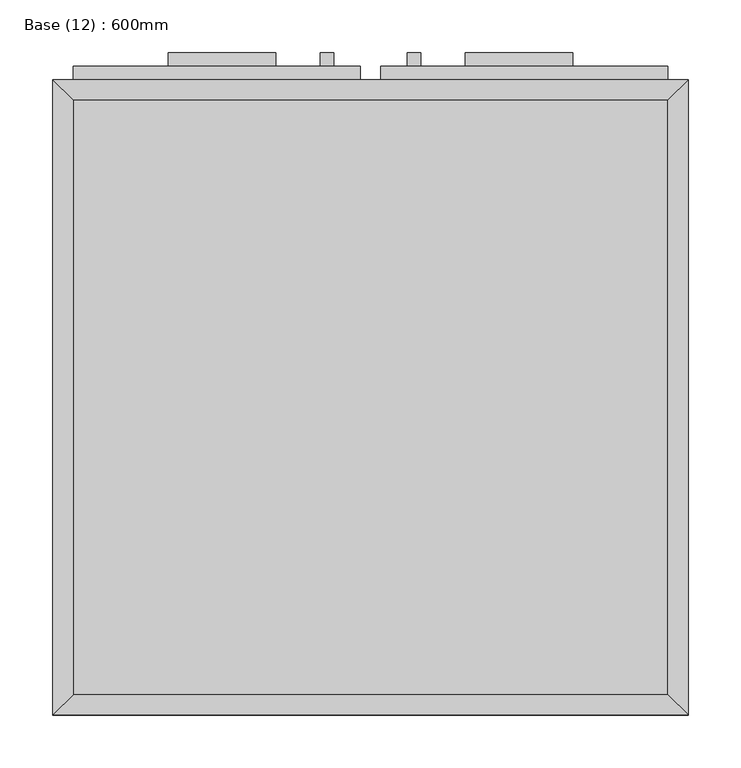
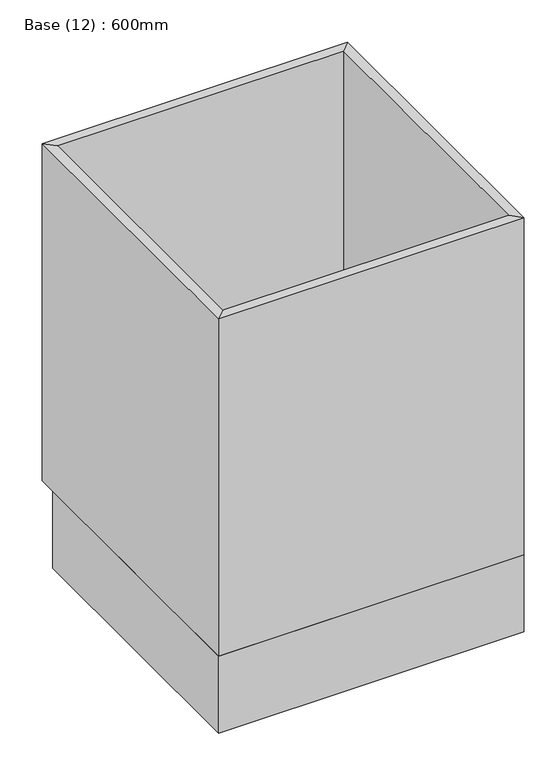
"""IFC4 building model written with IfcOpenShell, lengths in millimetres: furniture geometry, Base (12) : 600mm."""

import ifcopenshell
import ifcopenshell.guid

model = None  # the IFC model being written
_history = None  # IfcOwnerHistory: only IFC2X3 demands one
_inside = {}  # id of a spatial element -> (the spatial element, [elements in it])
_under = {}  # id of a project, library or spatial element -> (it, [spatial elements below it])
_declared = {}  # id of a project -> (the project, [libraries it declares])
_typed = {}  # id of a type object -> (the type object, [elements of that type])
_made_of = {}  # id of a material, layer set ... -> (it, [elements and type objects made of it])


def new_model(schema):
    """Start an empty IFC model of exactly this schema.

    Asked for "IFC4X3", IfcOpenShell would pick the latest addendum, in which some entities
    have other attributes; the version numbers below select the first issue.
    IFC2X3 requires an IfcOwnerHistory on every rooted entity: one is made here for all.
    """
    global model, _history
    if schema == "IFC4X3":
        model = ifcopenshell.file(schema_version=(4, 3, 0, 0))
    else:
        model = ifcopenshell.file(schema=schema)
    _inside.clear()
    _under.clear()
    _declared.clear()
    _typed.clear()
    _made_of.clear()
    _history = None
    if model.schema == "IFC2X3":
        org = make("IfcOrganization", Name="unknown")
        user = make(
            "IfcPersonAndOrganization",
            ThePerson=make("IfcPerson", FamilyName="unknown"),
            TheOrganization=org,
        )
        app = make(
            "IfcApplication",
            ApplicationDeveloper=org,
            Version="unknown",
            ApplicationFullName="unknown",
            ApplicationIdentifier="unknown",
        )
        _history = make(
            "IfcOwnerHistory",
            OwningUser=user,
            OwningApplication=app,
            ChangeAction="ADDED",
            CreationDate=0,
        )
    return model


def make(cls, **values):
    """One entity of the class cls with the attributes given. An attribute that is None is left unset."""
    return model.create_entity(
        cls, **{name: value for name, value in values.items() if value is not None}
    )


def rooted(cls, **values):
    """An entity with a GlobalId (a new one), such as an element, a storey or a relation."""
    return make(cls, GlobalId=ifcopenshell.guid.new(), OwnerHistory=_history, **values)


def si_unit(unit_type, name, prefix=None):
    """IfcSIUnit, for example si_unit("LENGTHUNIT", "METRE", prefix="MILLI")."""
    return make("IfcSIUnit", UnitType=unit_type, Prefix=prefix, Name=name)


def assignment(units):
    """IfcUnitAssignment: the units of a project."""
    return None if units is None else make("IfcUnitAssignment", Units=units)


def point(xyz):
    """IfcCartesianPoint."""
    return None if xyz is None else make("IfcCartesianPoint", Coordinates=xyz)


def direction(xyz):
    """IfcDirection."""
    return None if xyz is None else make("IfcDirection", DirectionRatios=xyz)


def frame(location, z_axis=None, x_axis=None):
    """IfcAxis2Placement3D, a coordinate frame: its origin and axes. An axis left out is left unset."""
    return make(
        "IfcAxis2Placement3D",
        Location=point(location),
        Axis=direction(z_axis),
        RefDirection=direction(x_axis),
    )


def origin():
    """The frame at (0, 0, 0) with its axes left unset."""
    return frame((0.0, 0.0, 0.0))


def origin_with_axes():
    """The frame at (0, 0, 0) with the z axis (0, 0, 1) and the x axis (1, 0, 0) written out."""
    return frame((0.0, 0.0, 0.0), z_axis=(0.0, 0.0, 1.0), x_axis=(1.0, 0.0, 0.0))


def place(relative_to, where):
    """IfcLocalPlacement: puts the frame where relative to a parent placement (None: the world)."""
    return make(
        "IfcLocalPlacement", PlacementRelTo=relative_to, RelativePlacement=where
    )


def context(
    kind, dimensions, precision=None, world=None, true_north=None, identifier=None
):
    """IfcGeometricRepresentationContext, for example the 3D "Model" context."""
    return make(
        "IfcGeometricRepresentationContext",
        ContextIdentifier=identifier,
        ContextType=kind,
        CoordinateSpaceDimension=dimensions,
        Precision=precision,
        WorldCoordinateSystem=world,
        TrueNorth=true_north,
    )


def project(units=None, contexts=None):
    """IfcProject with its units and contexts."""
    return rooted(
        "IfcProject",
        Name="project",
        RepresentationContexts=contexts,
        UnitsInContext=assignment(units),
    )


def spatial(cls, under=None, at=None, **own):
    """A site, building, storey or space (cls), placed at a placement, below another one or the project."""
    s = rooted(cls, ObjectPlacement=at, **own)
    if under is not None:
        _under.setdefault(under.id(), (under, []))[1].append(s)
    return s


def polyline(points):
    """IfcPolyline through the points."""
    return make("IfcPolyline", Points=[point(p) for p in points])


def outline(outer, holes=None, kind="AREA"):
    """IfcArbitraryClosedProfileDef: a profile drawn as a closed curve; with holes, ...WithVoids."""
    if holes is None:
        return make("IfcArbitraryClosedProfileDef", ProfileType=kind, OuterCurve=outer)
    return make(
        "IfcArbitraryProfileDefWithVoids",
        ProfileType=kind,
        OuterCurve=outer,
        InnerCurves=holes,
    )


def extrude(swept, where, along, depth):
    """IfcExtrudedAreaSolid: the profile swept, set in the frame where, extruded along a direction by depth."""
    return make(
        "IfcExtrudedAreaSolid",
        SweptArea=swept,
        Position=where,
        ExtrudedDirection=direction(along),
        Depth=depth,
    )


def faces_of(points, faces, orient=None, outer=None):
    """IfcFace entities. A face is a list of loops; a loop is a list of indices into points, from 0.

    orient and outer hold one flag for each loop. By default every Orientation is true, the
    first loop of a face is its IfcFaceOuterBound and the others are IfcFaceBound.
    """
    made = []
    for i, loops in enumerate(faces):
        bounds = []
        for j, loop in enumerate(loops):
            is_outer = j == 0 if outer is None else outer[i][j]
            bounds.append(
                make(
                    "IfcFaceOuterBound" if is_outer else "IfcFaceBound",
                    Bound=make("IfcPolyLoop", Polygon=[points[k] for k in loop]),
                    Orientation=True if orient is None else orient[i][j],
                )
            )
        made.append(make("IfcFace", Bounds=bounds))
    return made


def faceted_brep(points, faces, orient=None, outer=None, voids=None):
    """IfcFacetedBrep: a solid bounded by flat faces; with voids (closed shells), ...WithVoids."""
    shared = [point(p) for p in points]
    hull = make("IfcClosedShell", CfsFaces=faces_of(shared, faces, orient, outer))
    if voids is None:
        return make("IfcFacetedBrep", Outer=hull)
    return make(
        "IfcFacetedBrepWithVoids",
        Outer=hull,
        Voids=[
            make(cls, CfsFaces=faces_of(shared, fs, o, b)) for cls, fs, o, b in voids
        ],
    )


def shape(context_of_items, identifier, shape_type, items):
    """IfcShapeRepresentation: the items that make up one representation, for example the "Body"."""
    return make(
        "IfcShapeRepresentation",
        ContextOfItems=context_of_items,
        RepresentationIdentifier=identifier,
        RepresentationType=shape_type,
        Items=items,
    )


def source(mapping_origin, context_of_items, identifier, shape_type, items):
    """IfcRepresentationMap: a shape defined once, which mapped items show again and again."""
    return make(
        "IfcRepresentationMap",
        MappingOrigin=mapping_origin,
        MappedRepresentation=shape(context_of_items, identifier, shape_type, items),
    )


def transform(
    local_origin,
    x_axis=None,
    y_axis=None,
    z_axis=None,
    scale=None,
    scale2=None,
    scale3=None,
    uniform=True,
):
    """IfcCartesianTransformationOperator3D, or its non-uniform kind. x_axis, y_axis, z_axis: its Axis1, 2, 3."""
    if uniform:
        return make(
            "IfcCartesianTransformationOperator3D",
            Axis1=direction(x_axis),
            Axis2=direction(y_axis),
            LocalOrigin=point(local_origin),
            Scale=scale,
            Axis3=direction(z_axis),
        )
    return make(
        "IfcCartesianTransformationOperator3DnonUniform",
        Axis1=direction(x_axis),
        Axis2=direction(y_axis),
        LocalOrigin=point(local_origin),
        Scale=scale,
        Axis3=direction(z_axis),
        Scale2=scale2,
        Scale3=scale3,
    )


def mapped(mapping_source, mapping_target):
    """IfcMappedItem: shows the shape of a source again, moved by a transform."""
    return make(
        "IfcMappedItem", MappingSource=mapping_source, MappingTarget=mapping_target
    )


def made_of(thing, what):
    """Note that an element or type object is made of a material, layer set ...; save() writes the relation."""
    if what is not None:
        _made_of.setdefault(what.id(), (what, []))[1].append(thing)
    return thing


def element(
    cls,
    number,
    at=None,
    inside=None,
    cuts=None,
    type_object=None,
    material=None,
    context=None,
    identifier="Body",
    shape_type=None,
    held_by="IfcProductDefinitionShape",
    body=None,
    shapes=None,
    **own,
):
    """One element of the class cls, such as IfcWall. Its Tag is "e" and its number.

    at: its placement. inside: the storey or other place that contains it. cuts: it is an
    opening in that element (IfcRelVoidsElement). A single representation is given by context,
    identifier, shape_type and body (its items); several are given by shapes. held_by: the class
    of the entity that holds the representations. save() writes the other relations.
    """
    e = rooted(cls, Tag="e%d" % number, ObjectPlacement=at, **own)
    if body is not None:
        shapes = [shape(context, identifier, shape_type, body)]
    if shapes is not None:
        e.Representation = make(held_by, Representations=shapes)
    if inside is not None:
        _inside.setdefault(inside.id(), (inside, []))[1].append(e)
    if cuts is not None:
        rooted(
            "IfcRelVoidsElement", RelatingBuildingElement=cuts, RelatedOpeningElement=e
        )
    if type_object is not None:
        _typed.setdefault(type_object.id(), (type_object, []))[1].append(e)
    return made_of(e, material)


def aggregate(whole, parts):
    """IfcRelAggregates: a whole, such as a stair, and the parts it consists of."""
    return rooted("IfcRelAggregates", RelatingObject=whole, RelatedObjects=parts)


def save(model, path):
    """Write the relations noted so far, then the file.

    IfcRelAggregates (storeys below a building ...), IfcRelContainedInSpatialStructure (elements
    in a storey), IfcRelDefinesByType, IfcRelAssociatesMaterial and IfcRelDeclares: one each for
    every whole, place, type object, material and project.
    """
    for whole, parts in _under.values():
        aggregate(whole, parts)
    for where, things in _inside.values():
        rooted(
            "IfcRelContainedInSpatialStructure",
            RelatedElements=things,
            RelatingStructure=where,
        )
    for kind, things in _typed.values():
        rooted("IfcRelDefinesByType", RelatedObjects=things, RelatingType=kind)
    for what, things in _made_of.values():
        rooted("IfcRelAssociatesMaterial", RelatedObjects=things, RelatingMaterial=what)
    for by, libraries in _declared.values():
        rooted("IfcRelDeclares", RelatingContext=by, RelatedDefinitions=libraries)
    model.write(path)


def base_12_600mm_73813d14(model_context):
    return source(origin(), model_context, "Body", "SolidModel", [
        extrude(outline(polyline([(299.6877049, 19.05), (-262.2122951, 19.05), (-262.2122951, 580.95), (299.6877049, 580.95), (299.6877049, 19.05)])), frame((0.0, 0.0, 160.0), z_axis=(0.0, 0.0, 1.0), x_axis=(1.0, 0.0, 0.0)), (0.0, 0.0, 1.0), 19.05),
        faceted_brep([(299.6877049, 580.95, 860.0), (-262.2122951, 580.95, 860.0), (-262.2122951, 580.95, 160.0), (299.6877049, 580.95, 160.0), (318.7377049, 600.0, 860.0), (-281.2622951, 600.0, 860.0), (318.7377049, 600.0, 160.0), (-281.2622951, 600.0, 160.0), (-262.2122951, 19.05, 860.0), (-262.2122951, 19.05, 160.0), (-281.2622951, 0.0, 860.0), (-281.2622951, 0.0, 160.0), (299.6877049, 19.05, 860.0), (299.6877049, 19.05, 160.0), (318.7377049, 0.0, 860.0), (318.7377049, 0.0, 160.0)], [[[0, 1, 2, 3]], [[4, 5, 1, 0]], [[6, 7, 5, 4]], [[3, 2, 7, 6]], [[1, 8, 9, 2]], [[5, 10, 8, 1]], [[7, 11, 10, 5]], [[2, 9, 11, 7]], [[8, 12, 13, 9]], [[10, 14, 12, 8]], [[11, 15, 14, 10]], [[9, 13, 15, 11]], [[12, 0, 3, 13]], [[14, 4, 0, 12]], [[15, 6, 4, 14]], [[13, 3, 6, 15]]]),
        extrude(outline(polyline([(318.7377049, 0.0), (-281.2622951, 0.0), (-281.2622951, 565.0), (318.7377049, 565.0), (318.7377049, 0.0)])), origin_with_axes(), (0.0, 0.0, 1.0), 160.0),
        extrude(outline(polyline([(-70.9372951, 625.4), (-70.9372951, 612.7), (-172.5372951, 612.7), (-172.5372951, 625.4), (-70.9372951, 625.4)])), frame((0.0, 0.0, 802.85), z_axis=(0.0, 0.0, 1.0), x_axis=(1.0, 0.0, 0.0)), (0.0, 0.0, 1.0), 12.7),
        extrude(outline(polyline([(210.0127049, 625.4), (210.0127049, 612.7), (108.4127049, 612.7), (108.4127049, 625.4), (210.0127049, 625.4)])), frame((0.0, 0.0, 802.85), z_axis=(0.0, 0.0, 1.0), x_axis=(1.0, 0.0, 0.0)), (0.0, 0.0, 1.0), 12.7),
        extrude(outline(polyline([(-16.1872951, 625.4), (-16.1872951, 612.7), (-28.8872951, 612.7), (-28.8872951, 625.4), (-16.1872951, 625.4)])), frame((0.0, 0.0, 580.6), z_axis=(0.0, 0.0, 1.0), x_axis=(1.0, 0.0, 0.0)), (0.0, 0.0, 1.0), 101.6),
        extrude(outline(polyline([(66.3627049, 625.4), (66.3627049, 612.7), (53.6627049, 612.7), (53.6627049, 625.4), (66.3627049, 625.4)])), frame((0.0, 0.0, 580.6), z_axis=(0.0, 0.0, 1.0), x_axis=(1.0, 0.0, 0.0)), (0.0, 0.0, 1.0), 101.6),
        extrude(outline(polyline([(9.2127049, 612.7), (9.2127049, 600.0), (-262.2122951, 600.0), (-262.2122951, 612.7), (9.2127049, 612.7)])), frame((0.0, 0.0, 739.35), z_axis=(0.0, 0.0, 1.0), x_axis=(1.0, 0.0, 0.0)), (0.0, 0.0, 1.0), 101.6),
        extrude(outline(polyline([(299.6877049, 612.7), (299.6877049, 600.0), (28.2627049, 600.0), (28.2627049, 612.7), (299.6877049, 612.7)])), frame((0.0, 0.0, 739.35), z_axis=(0.0, 0.0, 1.0), x_axis=(1.0, 0.0, 0.0)), (0.0, 0.0, 1.0), 101.6),
        extrude(outline(polyline([(9.2127049, 612.7), (9.2127049, 600.0), (-262.2122951, 600.0), (-262.2122951, 612.7), (9.2127049, 612.7)])), frame((0.0, 0.0, 179.05), z_axis=(0.0, 0.0, 1.0), x_axis=(1.0, 0.0, 0.0)), (0.0, 0.0, 1.0), 541.25),
        extrude(outline(polyline([(299.6877049, 612.7), (299.6877049, 600.0), (28.2627049, 600.0), (28.2627049, 612.7), (299.6877049, 612.7)])), frame((0.0, 0.0, 179.05), z_axis=(0.0, 0.0, 1.0), x_axis=(1.0, 0.0, 0.0)), (0.0, 0.0, 1.0), 541.25),
    ])


if __name__ == "__main__":
    model = new_model("IFC4")
    model_context = context("Model", 3, world=origin())
    ifc_project = project(units=[si_unit("LENGTHUNIT", "METRE", prefix="MILLI")], contexts=[model_context])
    site = spatial("IfcSite", under=ifc_project)
    building = spatial("IfcBuilding", under=site)
    placement = place(None, origin())
    base_12_600mm_shape = base_12_600mm_73813d14(model_context)
    element("IfcFurniture", 1, ObjectType="Base (12) : 600mm", at=placement, inside=building, context=model_context, shape_type="MappedRepresentation", body=[
        mapped(base_12_600mm_shape, transform((0.0, 0.0, 0.0), x_axis=(1.0, 0.0, 0.0), y_axis=(0.0, 1.0, 0.0), z_axis=(0.0, 0.0, 1.0))),
    ])
    save(model, "model.ifc")

# Revit data of these elements
# Type "Base (12) : 600mm"
#   Keynote = "N10"
#   Depth = 600 mm
#   Height = 860 mm
#   Plinth Depth = 35 mm
#   Plinth Height = 160 mm
#   Width = 600 mm
#   Material Cabinet = Cabinets
#   Material Door/Drawer = Cabinets
#   Material Handle = Cabinets - Handles
#   Default Elevation = 0
# Element 1 (IfcFurniture, "Base (12) : 600mm")
#   Materials on its faces: "Cabinets", "Cabinets - Handles"
# Materials
#   "Cabinets": class "Miscellaneous", colour RGB 249 249 249, transparency 0
#   "Cabinets - Handles": class "Metal", colour RGB 57 57 57, transparency 0
